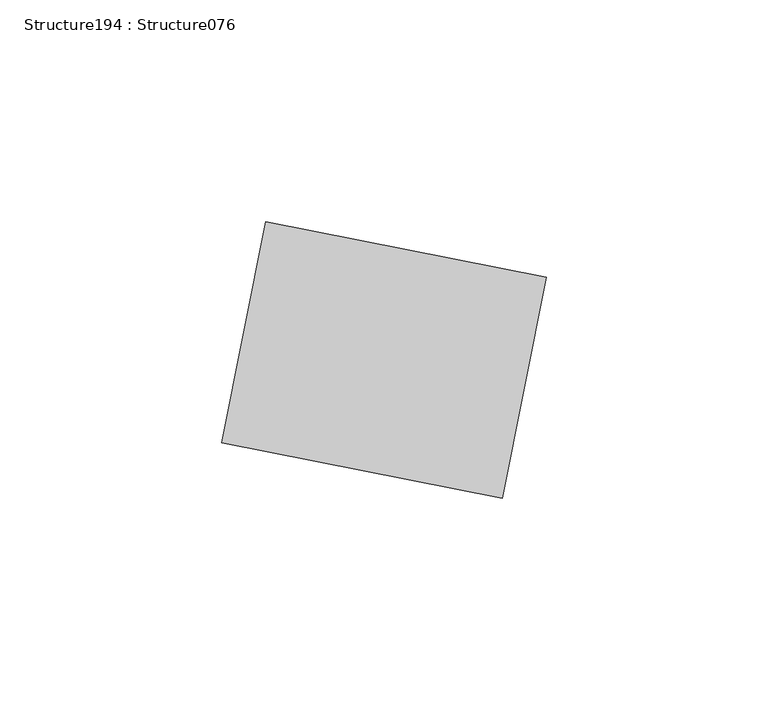
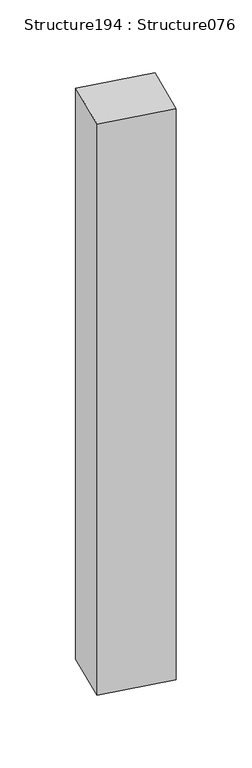
"""IFC4 building model written with IfcOpenShell, lengths in millimetres: proxy geometry, Structure194 : Structure076."""

from ifc_helpers import new_model, si_unit, frame, origin, place, context, project, spatial, polyline, outline, extrude, source, transform, mapped, element, save


def structure194_structure076_632d73ce(model_context):
    return source(origin(), model_context, "Body", "SweptSolid", [
        extrude(outline(polyline([(-2654.4961862, 235047.0764071), (-2591.1897674, 235034.5126994), (-2601.0786083, 234984.6844862), (-2664.3850271, 234997.2481939), (-2654.4961862, 235047.0764071)])), frame((0.0, 0.0, 595.2038833), z_axis=(0.0, 0.0, 1.0), x_axis=(1.0, 0.0, 0.0)), (0.0, 0.0, 1.0), 537.7810299),
    ])


if __name__ == "__main__":
    model = new_model("IFC4")
    model_context = context("Model", 3, world=origin())
    ifc_project = project(units=[si_unit("LENGTHUNIT", "METRE", prefix="MILLI")], contexts=[model_context])
    site = spatial("IfcSite", under=ifc_project)
    building = spatial("IfcBuilding", under=site)
    placement = place(None, origin())
    structure194_structure076_shape = structure194_structure076_632d73ce(model_context)
    element("IfcBuildingElementProxy", 1, Name="Structure194 : Structure076", ObjectType="Structure194 : Structure076", at=placement, inside=building, context=model_context, shape_type="MappedRepresentation", body=[
        mapped(structure194_structure076_shape, transform((0.0, 0.0, 0.0), x_axis=(1.0, 0.0, 0.0), y_axis=(0.0, 1.0, 0.0), z_axis=(0.0, 0.0, 1.0))),
    ])
    save(model, "model.ifc")

# Revit data of these elements
# Type "Structure194 : Structure076"
#   NameOverride = "Structure076"
# Element 1 (IfcBuildingElementProxy, "Structure194 : Structure076")
#   Materials on its faces: "BRUSHED ALUMINUM LETTERING"
# Materials
#   "BRUSHED ALUMINUM LETTERING": class "Unassigned", colour RGB 169 181 186, transparency 0, Cost = 0
